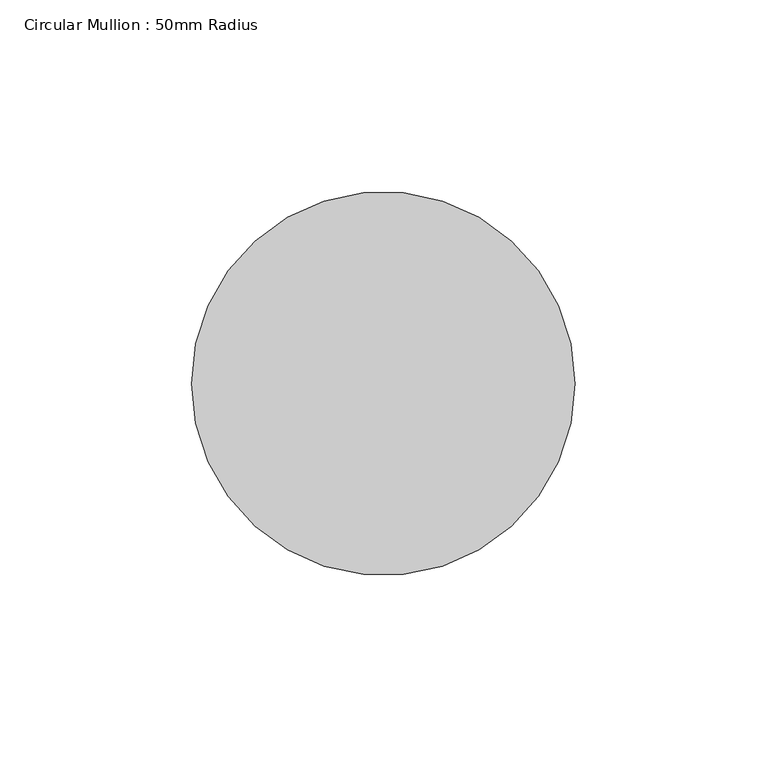
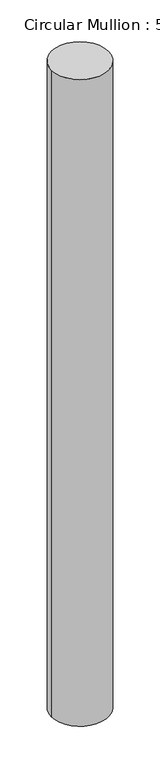
"""IFC4 building model written with IfcOpenShell, lengths in millimetres: member geometry, Circular Mullion : 50mm Radius."""

import ifcopenshell
import ifcopenshell.guid

model = None  # the IFC model being written
_history = None  # IfcOwnerHistory: only IFC2X3 demands one
_inside = {}  # id of a spatial element -> (the spatial element, [elements in it])
_under = {}  # id of a project, library or spatial element -> (it, [spatial elements below it])
_declared = {}  # id of a project -> (the project, [libraries it declares])
_typed = {}  # id of a type object -> (the type object, [elements of that type])
_made_of = {}  # id of a material, layer set ... -> (it, [elements and type objects made of it])


def new_model(schema):
    """Start an empty IFC model of exactly this schema.

    Asked for "IFC4X3", IfcOpenShell would pick the latest addendum, in which some entities
    have other attributes; the version numbers below select the first issue.
    IFC2X3 requires an IfcOwnerHistory on every rooted entity: one is made here for all.
    """
    global model, _history
    if schema == "IFC4X3":
        model = ifcopenshell.file(schema_version=(4, 3, 0, 0))
    else:
        model = ifcopenshell.file(schema=schema)
    _inside.clear()
    _under.clear()
    _declared.clear()
    _typed.clear()
    _made_of.clear()
    _history = None
    if model.schema == "IFC2X3":
        org = make("IfcOrganization", Name="unknown")
        user = make(
            "IfcPersonAndOrganization",
            ThePerson=make("IfcPerson", FamilyName="unknown"),
            TheOrganization=org,
        )
        app = make(
            "IfcApplication",
            ApplicationDeveloper=org,
            Version="unknown",
            ApplicationFullName="unknown",
            ApplicationIdentifier="unknown",
        )
        _history = make(
            "IfcOwnerHistory",
            OwningUser=user,
            OwningApplication=app,
            ChangeAction="ADDED",
            CreationDate=0,
        )
    return model


def make(cls, **values):
    """One entity of the class cls with the attributes given. An attribute that is None is left unset."""
    return model.create_entity(
        cls, **{name: value for name, value in values.items() if value is not None}
    )


def rooted(cls, **values):
    """An entity with a GlobalId (a new one), such as an element, a storey or a relation."""
    return make(cls, GlobalId=ifcopenshell.guid.new(), OwnerHistory=_history, **values)


def si_unit(unit_type, name, prefix=None):
    """IfcSIUnit, for example si_unit("LENGTHUNIT", "METRE", prefix="MILLI")."""
    return make("IfcSIUnit", UnitType=unit_type, Prefix=prefix, Name=name)


def assignment(units):
    """IfcUnitAssignment: the units of a project."""
    return None if units is None else make("IfcUnitAssignment", Units=units)


def point(xyz):
    """IfcCartesianPoint."""
    return None if xyz is None else make("IfcCartesianPoint", Coordinates=xyz)


def direction(xyz):
    """IfcDirection."""
    return None if xyz is None else make("IfcDirection", DirectionRatios=xyz)


def frame(location, z_axis=None, x_axis=None):
    """IfcAxis2Placement3D, a coordinate frame: its origin and axes. An axis left out is left unset."""
    return make(
        "IfcAxis2Placement3D",
        Location=point(location),
        Axis=direction(z_axis),
        RefDirection=direction(x_axis),
    )


def frame_2d(location, x_axis=None):
    """IfcAxis2Placement2D, a coordinate frame in the plane: its origin and x axis."""
    return make(
        "IfcAxis2Placement2D", Location=point(location), RefDirection=direction(x_axis)
    )


def origin():
    """The frame at (0, 0, 0) with its axes left unset."""
    return frame((0.0, 0.0, 0.0))


def origin_2d():
    """The frame at (0, 0) in the plane with its x axis left unset."""
    return frame_2d((0.0, 0.0))


def place(relative_to, where):
    """IfcLocalPlacement: puts the frame where relative to a parent placement (None: the world)."""
    return make(
        "IfcLocalPlacement", PlacementRelTo=relative_to, RelativePlacement=where
    )


def context(
    kind, dimensions, precision=None, world=None, true_north=None, identifier=None
):
    """IfcGeometricRepresentationContext, for example the 3D "Model" context."""
    return make(
        "IfcGeometricRepresentationContext",
        ContextIdentifier=identifier,
        ContextType=kind,
        CoordinateSpaceDimension=dimensions,
        Precision=precision,
        WorldCoordinateSystem=world,
        TrueNorth=true_north,
    )


def project(units=None, contexts=None):
    """IfcProject with its units and contexts."""
    return rooted(
        "IfcProject",
        Name="project",
        RepresentationContexts=contexts,
        UnitsInContext=assignment(units),
    )


def spatial(cls, under=None, at=None, **own):
    """A site, building, storey or space (cls), placed at a placement, below another one or the project."""
    s = rooted(cls, ObjectPlacement=at, **own)
    if under is not None:
        _under.setdefault(under.id(), (under, []))[1].append(s)
    return s


def circle_curve(where, radius):
    """IfcCircle in the frame where."""
    return make("IfcCircle", Position=where, Radius=radius)


def trimmed(basis, trim1, trim2, sense, master):
    """IfcTrimmedCurve: the piece of a basis curve between two trims."""
    return make(
        "IfcTrimmedCurve",
        BasisCurve=basis,
        Trim1=trim1,
        Trim2=trim2,
        SenseAgreement=sense,
        MasterRepresentation=master,
    )


def segment(curve, same_sense, transition):
    """IfcCompositeCurveSegment."""
    return make(
        "IfcCompositeCurveSegment",
        Transition=transition,
        SameSense=same_sense,
        ParentCurve=curve,
    )


def composite_curve(segments, self_intersect=None):
    """IfcCompositeCurve: segments joined end to end."""
    return make("IfcCompositeCurve", Segments=segments, SelfIntersect=self_intersect)


def outline(outer, holes=None, kind="AREA"):
    """IfcArbitraryClosedProfileDef: a profile drawn as a closed curve; with holes, ...WithVoids."""
    if holes is None:
        return make("IfcArbitraryClosedProfileDef", ProfileType=kind, OuterCurve=outer)
    return make(
        "IfcArbitraryProfileDefWithVoids",
        ProfileType=kind,
        OuterCurve=outer,
        InnerCurves=holes,
    )


def extrude(swept, where, along, depth):
    """IfcExtrudedAreaSolid: the profile swept, set in the frame where, extruded along a direction by depth."""
    return make(
        "IfcExtrudedAreaSolid",
        SweptArea=swept,
        Position=where,
        ExtrudedDirection=direction(along),
        Depth=depth,
    )


def shape(context_of_items, identifier, shape_type, items):
    """IfcShapeRepresentation: the items that make up one representation, for example the "Body"."""
    return make(
        "IfcShapeRepresentation",
        ContextOfItems=context_of_items,
        RepresentationIdentifier=identifier,
        RepresentationType=shape_type,
        Items=items,
    )


def source(mapping_origin, context_of_items, identifier, shape_type, items):
    """IfcRepresentationMap: a shape defined once, which mapped items show again and again."""
    return make(
        "IfcRepresentationMap",
        MappingOrigin=mapping_origin,
        MappedRepresentation=shape(context_of_items, identifier, shape_type, items),
    )


def transform(
    local_origin,
    x_axis=None,
    y_axis=None,
    z_axis=None,
    scale=None,
    scale2=None,
    scale3=None,
    uniform=True,
):
    """IfcCartesianTransformationOperator3D, or its non-uniform kind. x_axis, y_axis, z_axis: its Axis1, 2, 3."""
    if uniform:
        return make(
            "IfcCartesianTransformationOperator3D",
            Axis1=direction(x_axis),
            Axis2=direction(y_axis),
            LocalOrigin=point(local_origin),
            Scale=scale,
            Axis3=direction(z_axis),
        )
    return make(
        "IfcCartesianTransformationOperator3DnonUniform",
        Axis1=direction(x_axis),
        Axis2=direction(y_axis),
        LocalOrigin=point(local_origin),
        Scale=scale,
        Axis3=direction(z_axis),
        Scale2=scale2,
        Scale3=scale3,
    )


def mapped(mapping_source, mapping_target):
    """IfcMappedItem: shows the shape of a source again, moved by a transform."""
    return make(
        "IfcMappedItem", MappingSource=mapping_source, MappingTarget=mapping_target
    )


def made_of(thing, what):
    """Note that an element or type object is made of a material, layer set ...; save() writes the relation."""
    if what is not None:
        _made_of.setdefault(what.id(), (what, []))[1].append(thing)
    return thing


def element(
    cls,
    number,
    at=None,
    inside=None,
    cuts=None,
    type_object=None,
    material=None,
    context=None,
    identifier="Body",
    shape_type=None,
    held_by="IfcProductDefinitionShape",
    body=None,
    shapes=None,
    **own,
):
    """One element of the class cls, such as IfcWall. Its Tag is "e" and its number.

    at: its placement. inside: the storey or other place that contains it. cuts: it is an
    opening in that element (IfcRelVoidsElement). A single representation is given by context,
    identifier, shape_type and body (its items); several are given by shapes. held_by: the class
    of the entity that holds the representations. save() writes the other relations.
    """
    e = rooted(cls, Tag="e%d" % number, ObjectPlacement=at, **own)
    if body is not None:
        shapes = [shape(context, identifier, shape_type, body)]
    if shapes is not None:
        e.Representation = make(held_by, Representations=shapes)
    if inside is not None:
        _inside.setdefault(inside.id(), (inside, []))[1].append(e)
    if cuts is not None:
        rooted(
            "IfcRelVoidsElement", RelatingBuildingElement=cuts, RelatedOpeningElement=e
        )
    if type_object is not None:
        _typed.setdefault(type_object.id(), (type_object, []))[1].append(e)
    return made_of(e, material)


def aggregate(whole, parts):
    """IfcRelAggregates: a whole, such as a stair, and the parts it consists of."""
    return rooted("IfcRelAggregates", RelatingObject=whole, RelatedObjects=parts)


def save(model, path):
    """Write the relations noted so far, then the file.

    IfcRelAggregates (storeys below a building ...), IfcRelContainedInSpatialStructure (elements
    in a storey), IfcRelDefinesByType, IfcRelAssociatesMaterial and IfcRelDeclares: one each for
    every whole, place, type object, material and project.
    """
    for whole, parts in _under.values():
        aggregate(whole, parts)
    for where, things in _inside.values():
        rooted(
            "IfcRelContainedInSpatialStructure",
            RelatedElements=things,
            RelatingStructure=where,
        )
    for kind, things in _typed.values():
        rooted("IfcRelDefinesByType", RelatedObjects=things, RelatingType=kind)
    for what, things in _made_of.values():
        rooted("IfcRelAssociatesMaterial", RelatedObjects=things, RelatingMaterial=what)
    for by, libraries in _declared.values():
        rooted("IfcRelDeclares", RelatingContext=by, RelatedDefinitions=libraries)
    model.write(path)


def circular_mullion_50mm_radius_ab1d5612(model_context):
    return source(origin(), model_context, "Body", "SweptSolid", [
        extrude(outline(composite_curve([segment(trimmed(circle_curve(origin_2d(), 50.0), [point((50.0, 0.0))], [point((-50.0, 0.0))], False, "CARTESIAN"), True, "CONTINUOUS"), segment(trimmed(circle_curve(origin_2d(), 50.0), [point((-50.0, 0.0))], [point((50.0, 0.0))], False, "CARTESIAN"), True, "CONTINUOUS")], self_intersect=False)), frame((0.0, 0.0, -1198.0720807), z_axis=(0.0, 0.0, 1.0), x_axis=(1.0, 0.0, 0.0)), (0.0, 0.0, 1.0), 1198.0720807),
    ])


if __name__ == "__main__":
    model = new_model("IFC4")
    model_context = context("Model", 3, world=origin())
    ifc_project = project(units=[si_unit("LENGTHUNIT", "METRE", prefix="MILLI")], contexts=[model_context])
    site = spatial("IfcSite", under=ifc_project)
    building = spatial("IfcBuilding", under=site)
    placement = place(None, origin())
    circular_mullion_50mm_radius_shape = circular_mullion_50mm_radius_ab1d5612(model_context)
    element("IfcMember", 1, ObjectType="Circular Mullion : 50mm Radius", at=placement, inside=building, context=model_context, shape_type="MappedRepresentation", body=[
        mapped(circular_mullion_50mm_radius_shape, transform((0.0, 0.0, 0.0), x_axis=(1.0, 0.0, 0.0), y_axis=(0.0, 1.0, 0.0), z_axis=(0.0, 0.0, 1.0))),
    ])
    save(model, "model.ifc")

# Revit data of these elements
# Type "Circular Mullion : 50mm Radius"
#   built-in parameter 1007350 = 0.164042 (stored number, unit not read)
# Element 1 (IfcMember, "Circular Mullion : 50mm Radius")
#   Materials on its faces: "Aluminium"
# Materials
#   "Aluminium": class "Metal", colour RGB 247 247 247, transparency 0, Description = "Aluminium 6061", Cost = 0
